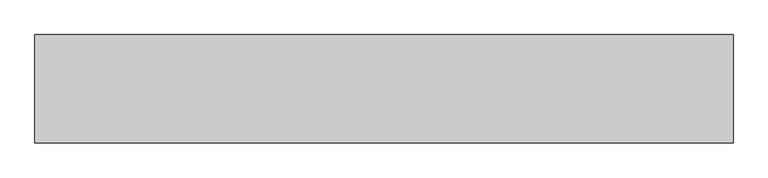
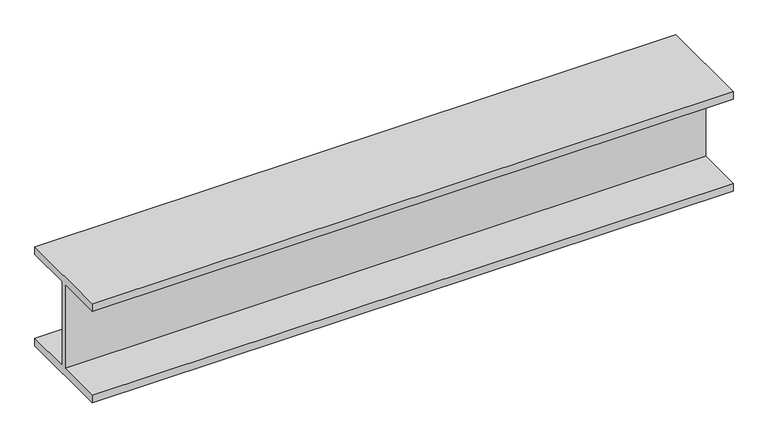
"""IFC4 building model written with IfcOpenShell, lengths in millimetres: proxy geometry, Structure053 5969 : Structure053 5969."""

from ifc_helpers import new_model, si_unit, frame, origin, place, context, project, spatial, polyline, outline, extrude, source, transform, mapped, element, save


def generic_models_5324979f(model_context):
    return source(origin(), model_context, "Body", "SweptSolid", [
        extrude(outline(polyline([(-4993.9300258, 40112.6960938), (-4993.9300258, 40087.5500938), (-5141.1205761, 40087.5500938), (-5141.1205761, 39810.1820937), (-4993.9300258, 39810.1820937), (-4993.9300258, 39785.0360937), (-5303.8100258, 39785.0360937), (-5303.8100258, 39810.182), (-5156.6145761, 39810.182), (-5156.6145761, 40087.5500938), (-5303.8100258, 40087.5500938), (-5303.8100258, 40112.6960938), (-4993.9300258, 40112.6960938)])), frame((254.64, 0.0, 0.0), z_axis=(1.0, 0.0, 0.0), x_axis=(0.0, 1.0, 0.0)), (0.0, 0.0, 1.0), 2000.25),
    ])


if __name__ == "__main__":
    model = new_model("IFC4")
    model_context = context("Model", 3, world=origin())
    ifc_project = project(units=[si_unit("LENGTHUNIT", "METRE", prefix="MILLI")], contexts=[model_context])
    site = spatial("IfcSite", under=ifc_project)
    building = spatial("IfcBuilding", under=site)
    placement = place(None, origin())
    generic_models_shape = generic_models_5324979f(model_context)
    element("IfcBuildingElementProxy", 1, Name="Structure053 5969 : Structure053 5969", ObjectType="Structure053 5969 : Structure053 5969", at=placement, inside=building, context=model_context, shape_type="MappedRepresentation", body=[
        mapped(generic_models_shape, transform((0.0, 0.0, 0.0), x_axis=(1.0, 0.0, 0.0), y_axis=(0.0, 1.0, 0.0), z_axis=(0.0, 0.0, 1.0))),
    ])
    save(model, "model.ifc")

# Revit data of these elements
# Type "Structure053 5969 : Structure053 5969"
#   NameOverride = "Structure053"
# Element 1 (IfcBuildingElementProxy, "Structure053 5969 : Structure053 5969")
#   Materials on its faces: "IfcSurfaceStyle #5964"
# Materials
#   "IfcSurfaceStyle #5964": class "Unassigned", colour RGB 150 169 186, transparency 0
